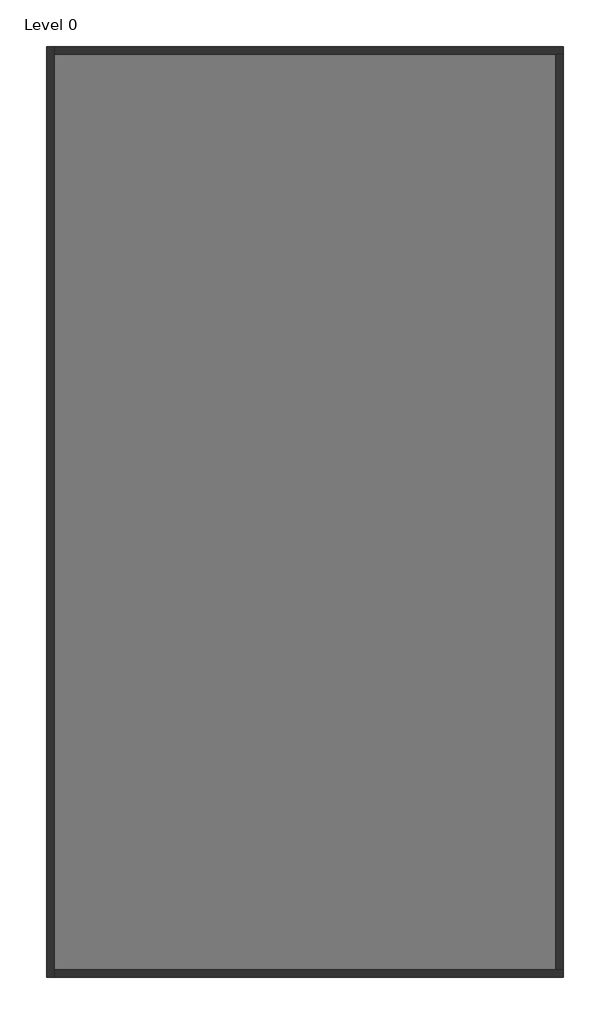
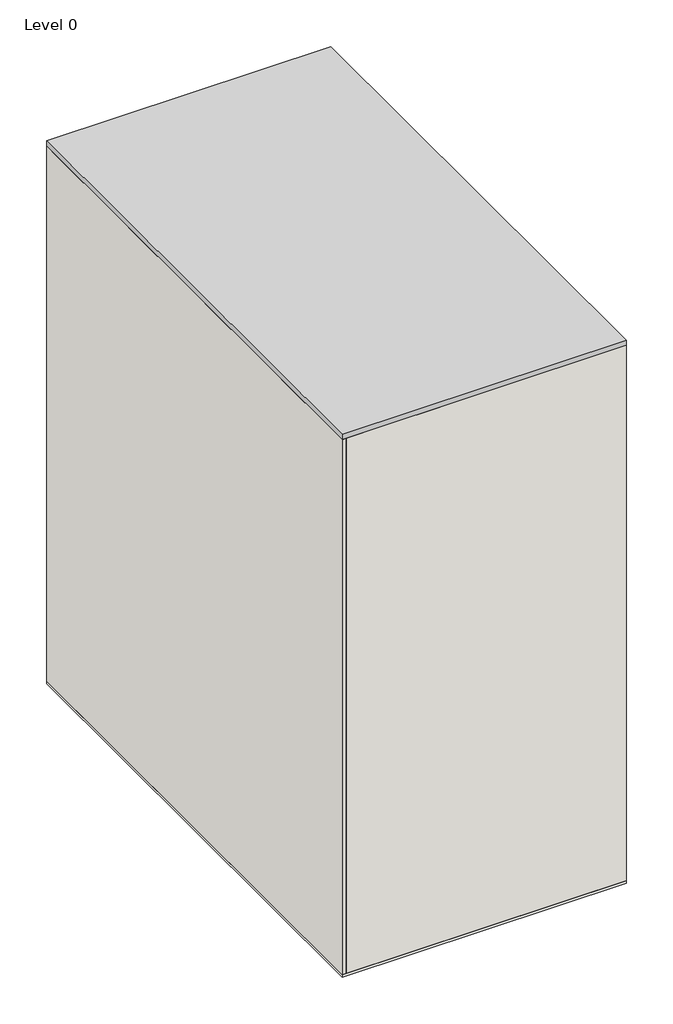
# One storey: 4 walls, 1 proxy, 1 slab.
"""IFC4 building model written with IfcOpenShell, lengths in millimetres."""

from ifc_helpers import new_model, si_unit, frame, origin, origin_with_axes, place, context, project, spatial, polyline, outline, extrude, faceted_brep, element, save

model = new_model("IFC4")

# Units and contexts
model_context = context("Model", 3, world=origin())
ifc_project = project(units=[si_unit("LENGTHUNIT", "METRE", prefix="MILLI")], contexts=[model_context])

# Site, building, storey
site = spatial("IfcSite", under=ifc_project)
building = spatial("IfcBuilding", under=site)
storey = spatial("IfcBuildingStorey", under=building, Name="Level 0", Elevation=100.0)

# Proxy
placement = place(None, origin())
element("IfcBuildingElementProxy", 1, Name="LowUrbanDensityBuilding : LowUrbanDensityBuilding", ObjectType="LowUrbanDensityBuilding : LowUrbanDensityBuilding", at=placement, inside=storey, context=model_context, shape_type="SweptSolid", body=[
    extrude(outline(polyline([(7325.2659446, 3676.2074539), (7325.2659446, -14323.7925461), (-2674.7340554, -14323.7925461), (-2674.7340554, 3676.2074539), (7325.2659446, 3676.2074539)])), origin_with_axes(), (0.0, 0.0, 1.0), 20200.0),
])

# Slab
element("IfcSlab", 2, ObjectType="Floor-Concrete_100Con", at=placement, inside=storey, context=model_context, shape_type="SweptSolid", body=[
    extrude(outline(polyline([(7325.2659446, 3676.2074539), (7325.2659446, -14323.7925461), (-2674.7340554, -14323.7925461), (-2674.7340554, 3676.2074539), (7325.2659446, 3676.2074539)])), origin_with_axes(), (0.0, 0.0, 1.0), 100.0),
])

# Walls
element("IfcWall", 3, ObjectType="Wall-Ext_25Rdr-100Blk-19P", at=placement, inside=storey, context=model_context, shape_type="Brep", body=[
    faceted_brep([(-2674.7340554, 3676.2074539, 100.0), (-2674.7340554, -14323.7925461, 100.0), (-2674.7340554, -14323.7925461, 20000.0), (-2674.7340554, 3676.2074539, 20000.0), (-2530.4340554, 3676.2074539, 100.0), (-2530.4340554, 3676.2074539, 20000.0), (-2530.4340554, 3531.9074539, 20000.0), (-2530.4340554, -14179.4925461, 20000.0), (-2530.4340554, -14323.7925461, 20000.0), (-2530.4340554, -14323.7925461, 100.0), (-2530.4340554, -14179.4925461, 100.0), (-2530.4340554, 3531.9074539, 100.0)], [[[0, 1, 2, 3]], [[4, 5, 6, 7, 8, 9, 10, 11]], [[1, 0, 4, 11, 10, 9]], [[3, 2, 8, 7, 6, 5]], [[2, 1, 9, 8]], [[0, 3, 5, 4]]]),
])
element("IfcWall", 4, ObjectType="Wall-Ext_25Rdr-100Blk-19P", at=placement, inside=storey, context=model_context, shape_type="Brep", body=[
    faceted_brep([(-2530.4340554, -14323.7925461, 100.0), (7325.2659446, -14323.7925461, 100.0), (7325.2659446, -14323.7925461, 20000.0), (-2530.4340554, -14323.7925461, 20000.0), (-2530.4340554, -14179.4925461, 100.0), (-2530.4340554, -14179.4925461, 20000.0), (7180.9659446, -14179.4925461, 20000.0), (7325.2659446, -14179.4925461, 20000.0), (7325.2659446, -14179.4925461, 100.0), (7180.9659446, -14179.4925461, 100.0)], [[[0, 1, 2, 3]], [[4, 5, 6, 7, 8, 9]], [[1, 0, 4, 9, 8]], [[3, 2, 7, 6, 5]], [[0, 3, 5, 4]], [[2, 1, 8, 7]]]),
])
element("IfcWall", 5, ObjectType="Wall-Ext_25Rdr-100Blk-19P", at=placement, inside=storey, context=model_context, shape_type="Brep", body=[
    faceted_brep([(7325.2659446, 3676.2074539, 100.0), (-2530.4340554, 3676.2074539, 100.0), (-2530.4340554, 3676.2074539, 20000.0), (7325.2659446, 3676.2074539, 20000.0), (7325.2659446, 3531.9074539, 100.0), (7325.2659446, 3531.9074539, 20000.0), (7180.9659446, 3531.9074539, 20000.0), (-2530.4340554, 3531.9074539, 20000.0), (-2530.4340554, 3531.9074539, 100.0), (7180.9659446, 3531.9074539, 100.0)], [[[0, 1, 2, 3]], [[4, 5, 6, 7, 8, 9]], [[1, 0, 4, 9, 8]], [[3, 2, 7, 6, 5]], [[2, 1, 8, 7]], [[0, 3, 5, 4]]]),
])
element("IfcWall", 6, ObjectType="Wall-Ext_25Rdr-100Blk-19P", at=placement, inside=storey, context=model_context, shape_type="SweptSolid", body=[
    extrude(outline(polyline([(7325.2659446, 3531.9074539), (7325.2659446, -14179.4925461), (7180.9659446, -14179.4925461), (7180.9659446, 3531.9074539), (7325.2659446, 3531.9074539)])), frame((0.0, 0.0, 100.0), z_axis=(0.0, 0.0, 1.0), x_axis=(1.0, 0.0, 0.0)), (0.0, 0.0, 1.0), 19900.0),
])

save(model, "model.ifc")

# Revit data of these elements
# Project information
#   Project Issue Date = "Issue Date"
#   Project Status = "Project Status"
#   Client Name = "Owner"
#   Project Address = "Enter address here"
#   Project Name = "Project Name"
#   Project Number = "Project Number"
# Type "Floor-Concrete_100Con"
#   Keynote = "E60/130"
#   Function = 0
#   Layers, outside or top first: 100 mm "Concrete" (function 1)
# Type "Wall-Ext_25Rdr-100Blk-19P"
#   Keynote = "F10"
#   Layers, outside or top first: 25.3 mm "Render, Beige, Smooth" (function 5); 100 mm "Concrete Masonry Units _Low Density" (function 1); 19 mm "Plaster" (function 5)
# Element 1 (IfcBuildingElementProxy, "LowUrbanDensityBuilding : LowUrbanDensityBuilding")
#   Phase Created = New Construction
#   Materials on its faces: "Default Form"
# Element 2 (IfcSlab, "Floor-Concrete_100Con")
#   Height Offset From Level = 0 mm
#   Phase Created = New Construction
#   Materials on its faces: "Concrete"
# Element 3 (IfcWall, "Wall-Ext_25Rdr-100Blk-19P")
#   Top Offset = 0 mm
#   Base Offset = 0 mm
#   wall height = 19900 mm
#   Phase Created = New Construction
#   Base Constraint = Level 0
#   Top Constraint = Level 5
#   Materials on its faces: "Render, Beige, Smooth", "Default Wall", "Plaster"
# Elements 4, 5, 6 (IfcWall, "Wall-Ext_25Rdr-100Blk-19P")
#   Top Offset = 0 mm
#   Base Offset = 0 mm
#   wall height = 19900 mm
#   Phase Created = New Construction
#   Base Constraint = Level 0
#   Top Constraint = Level 5
#   Materials on its faces: "Default Wall", "Render, Beige, Smooth", "Plaster"
# Materials
#   "Concrete": class "Concrete", colour RGB 120 120 120, transparency 0, Description = "Portland Cement Concrete", Cost = 0
#   "Render, Beige, Smooth": class "Generic", colour RGB 213 198 180, transparency 0, Description = "physical material", Cost = 0
#   "Concrete Masonry Units _Low Density": class "Masonry", colour RGB 181 181 181, transparency 0, Description = "Concrete masonry units", Cost = 0
#   "Plaster": class "Generic", colour RGB 249 249 249, transparency 0, Description = "Plaster", Cost = 0
#   "Default Form": class "Generic", colour RGB 185 189 196, transparency 0.5, Cost = 0
#   "Default Wall": class "Miscellaneous", colour RGB 128 128 128, transparency 0, Comments = "Rendering appearance not upgraded Rendering appearance not upgraded ", Cost = 0
